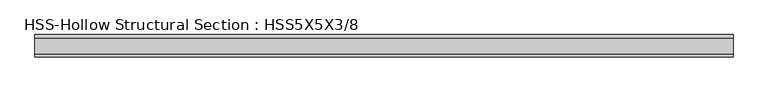
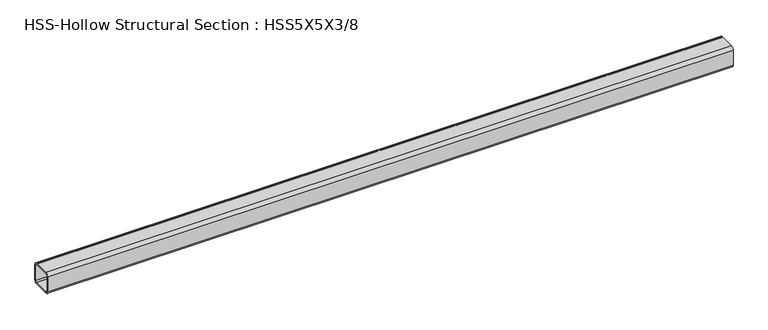
"""IFC4 building model written with IfcOpenShell, lengths in millimetres: member geometry, HSS-Hollow Structural Section : HSS5X5X3/8."""

from ifc_helpers import new_model, si_unit, point, frame, frame_2d, origin, place, context, project, spatial, polyline, circle_curve, trimmed, segment, composite_curve, outline, extrude, source, transform, mapped, element, save


def hss_hollow_structural_section_hss5x5x3_8_6a13ed6b(model_context):
    return source(origin(), model_context, "Body", "SweptSolid", [
        extrude(outline(composite_curve([segment(polyline([(63.5, 45.7708), (63.5, -45.7708)]), True, "CONTINUOUS"), segment(trimmed(circle_curve(frame_2d((45.7708, -45.7708)), 17.7292), [point((63.5, -45.7708))], [point((45.7708, -63.5))], False, "CARTESIAN"), True, "CONTINUOUS"), segment(polyline([(45.7708, -63.5), (-45.7708, -63.5)]), True, "CONTINUOUS"), segment(trimmed(circle_curve(frame_2d((-45.7708, -45.7708)), 17.7292), [point((-45.7708, -63.5))], [point((-63.5, -45.7708))], False, "CARTESIAN"), True, "CONTINUOUS"), segment(polyline([(-63.5, -45.7708), (-63.5, 45.7708)]), True, "CONTINUOUS"), segment(trimmed(circle_curve(frame_2d((-45.7708, 45.7708)), 17.7292), [point((-63.5, 45.7708))], [point((-45.7708, 63.5))], False, "CARTESIAN"), True, "CONTINUOUS"), segment(polyline([(-45.7708, 63.5), (45.7708, 63.5)]), True, "CONTINUOUS"), segment(trimmed(circle_curve(frame_2d((45.7708, 45.7708)), 17.7292), [point((45.7708, 63.5))], [point((63.5, 45.7708))], False, "CARTESIAN"), True, "CONTINUOUS")], self_intersect=False), holes=[composite_curve([segment(trimmed(circle_curve(frame_2d((-45.7708, 45.7708)), 8.8646), [point((-45.7708, 54.6354))], [point((-54.6354, 45.7708))], True, "CARTESIAN"), True, "CONTINUOUS"), segment(polyline([(-54.6354, 45.7708), (-54.6354, -45.7708)]), True, "CONTINUOUS"), segment(trimmed(circle_curve(frame_2d((-45.7708, -45.7708)), 8.8646), [point((-54.6354, -45.7708))], [point((-45.7708, -54.6354))], True, "CARTESIAN"), True, "CONTINUOUS"), segment(polyline([(-45.7708, -54.6354), (45.7708, -54.6354)]), True, "CONTINUOUS"), segment(trimmed(circle_curve(frame_2d((45.7708, -45.7708)), 8.8646), [point((45.7708, -54.6354))], [point((54.6354, -45.7708))], True, "CARTESIAN"), True, "CONTINUOUS"), segment(polyline([(54.6354, -45.7708), (54.6354, 45.7708)]), True, "CONTINUOUS"), segment(trimmed(circle_curve(frame_2d((45.7708, 45.7708)), 8.8646), [point((54.6354, 45.7708))], [point((45.7708, 54.6354))], True, "CARTESIAN"), True, "CONTINUOUS"), segment(polyline([(45.7708, 54.6354), (-45.7708, 54.6354)]), True, "CONTINUOUS")], self_intersect=False)]), frame((-1992.0366425, 0.0, 0.0), z_axis=(1.0, 0.0, 0.0), x_axis=(0.0, 1.0, 0.0)), (0.0, 0.0, 1.0), 3984.0732849),
    ])


if __name__ == "__main__":
    model = new_model("IFC4")
    model_context = context("Model", 3, world=origin())
    ifc_project = project(units=[si_unit("LENGTHUNIT", "METRE", prefix="MILLI")], contexts=[model_context])
    site = spatial("IfcSite", under=ifc_project)
    building = spatial("IfcBuilding", under=site)
    placement = place(None, origin())
    hss_hollow_structural_section_hss5x5x3_8_shape = hss_hollow_structural_section_hss5x5x3_8_6a13ed6b(model_context)
    element("IfcMember", 1, ObjectType="HSS-Hollow Structural Section : HSS5X5X3/8", at=placement, inside=building, context=model_context, shape_type="MappedRepresentation", body=[
        mapped(hss_hollow_structural_section_hss5x5x3_8_shape, transform((0.0, 0.0, 0.0), x_axis=(1.0, 0.0, 0.0), y_axis=(0.0, 1.0, 0.0), z_axis=(0.0, 0.0, 1.0))),
    ])
    save(model, "model.ifc")

# Revit data of these elements
# Type "HSS-Hollow Structural Section : HSS5X5X3/8"
#   Assembly Code = "B10"
#   Shape = "Square"
#   W = 22.3
#   Ht = 0' - 5"
#   Length [instance default] = 5' - 0"
#   b = 0' - 5"
#   kr = 0' - 0.698"
#   t = 0' - 0.349"
#   A = 0.0429167 SF
#   Structural Material [instance default] = Steel ASTM A500, Grade B, Rectangular and Square
# Element 1 (IfcMember, "HSS-Hollow Structural Section : HSS5X5X3/8")
#   Materials on its faces: "Steel ASTM A500, Grade B, Rectangular and Square"
# Materials
#   "Steel ASTM A500, Grade B, Rectangular and Square": class "Metal", colour RGB 199 199 199, transparency 0, Description = "Carbon steel", Cost = 0
